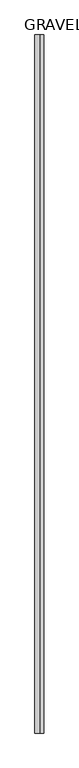
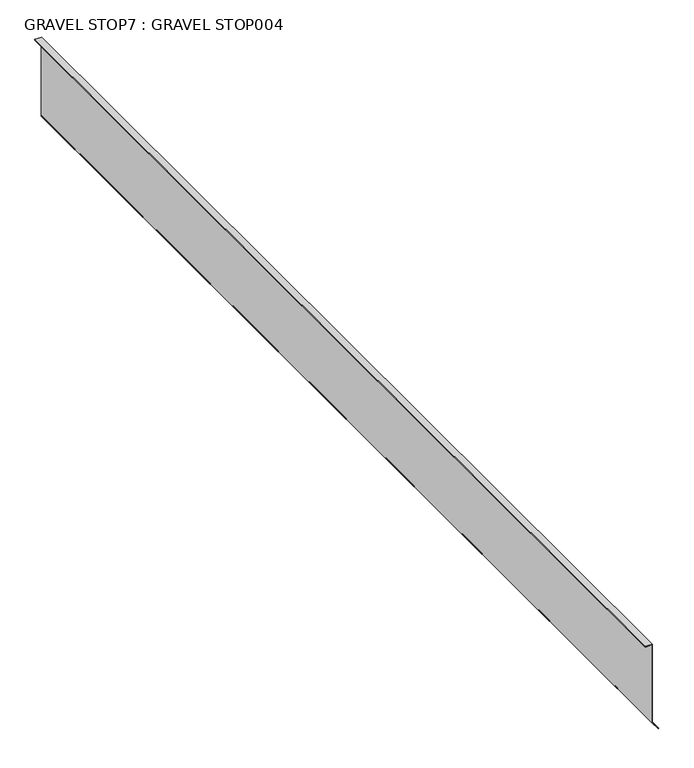
"""IFC4 building model written with IfcOpenShell, lengths in millimetres: proxy geometry, GRAVEL STOP7 : GRAVEL STOP004."""

from ifc_helpers import new_model, si_unit, frame, origin, place, context, project, spatial, polyline, outline, extrude, source, transform, mapped, element, save


def gravel_stop7_gravel_stop004_78d96abb(model_context):
    return source(origin(), model_context, "Body", "SweptSolid", [
        extrude(outline(polyline([(40082.2407116, -4352.793241), (40097.9858473, -4365.3568119), (40254.7357103, -4365.3568119), (40254.7357103, -4378.5358417), (40253.3245993, -4378.5358417), (40253.3245993, -4366.7679229), (40097.4918556, -4366.7679229), (40081.3605882, -4353.8962446), (40082.2407116, -4352.793241)])), frame((0.0, -1065.5906573, 0.0), z_axis=(0.0, 1.0, 0.0), x_axis=(0.0, 0.0, 1.0)), (0.0, 0.0, 1.0), 2000.25),
    ])


if __name__ == "__main__":
    model = new_model("IFC4")
    model_context = context("Model", 3, world=origin())
    ifc_project = project(units=[si_unit("LENGTHUNIT", "METRE", prefix="MILLI")], contexts=[model_context])
    site = spatial("IfcSite", under=ifc_project)
    building = spatial("IfcBuilding", under=site)
    placement = place(None, origin())
    gravel_stop7_gravel_stop004_shape = gravel_stop7_gravel_stop004_78d96abb(model_context)
    element("IfcBuildingElementProxy", 1, Name="GRAVEL STOP7 : GRAVEL STOP004", ObjectType="GRAVEL STOP7 : GRAVEL STOP004", at=placement, inside=building, context=model_context, shape_type="MappedRepresentation", body=[
        mapped(gravel_stop7_gravel_stop004_shape, transform((0.0, 0.0, 0.0), x_axis=(1.0, 0.0, 0.0), y_axis=(0.0, 1.0, 0.0), z_axis=(0.0, 0.0, 1.0))),
    ])
    save(model, "model.ifc")

# Revit data of these elements
# Type "GRAVEL STOP7 : GRAVEL STOP004"
#   NameOverride = "GRAVEL STOP004"
# Element 1 (IfcBuildingElementProxy, "GRAVEL STOP7 : GRAVEL STOP004")
#   Materials on its faces: "GRAVEL STOP REQUIRED WITH GRAVEL SURFACE SYSTEMS"
# Materials
#   "GRAVEL STOP REQUIRED WITH GRAVEL SURFACE SYSTEMS": class "Unassigned", colour RGB 170 170 127, transparency 0, Cost = 0
